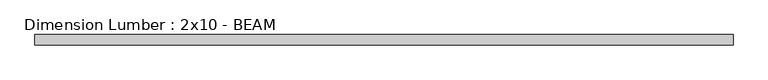
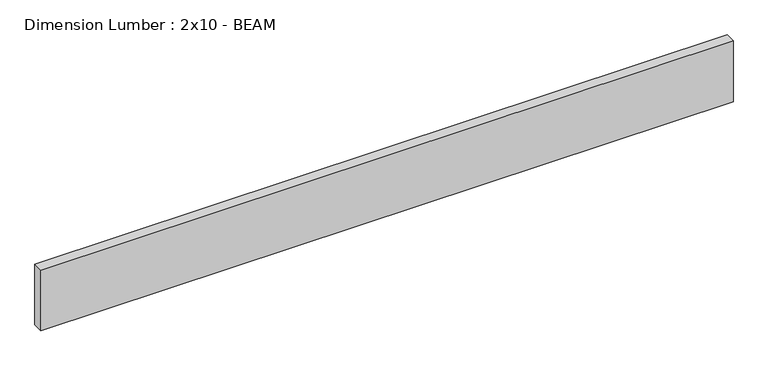
"""IFC4 building model written with IfcOpenShell, lengths in millimetres: beam geometry, Dimension Lumber : 2x10 - BEAM."""

from ifc_helpers import new_model, si_unit, frame, origin, place, context, project, spatial, polyline, outline, extrude, source, transform, mapped, element, save


def dimension_lumber_2x10_beam_c97c06ab(model_context):
    return source(origin(), model_context, "Body", "SweptSolid", [
        extrude(outline(polyline([(1213.64375, 19.05), (1213.64375, -19.05), (-1323.18125, -19.05), (-1323.18125, 19.05), (1213.64375, 19.05)])), frame((0.0, 0.0, -117.475), z_axis=(0.0, 0.0, 1.0), x_axis=(1.0, 0.0, 0.0)), (0.0, 0.0, 1.0), 234.95),
    ])


if __name__ == "__main__":
    model = new_model("IFC4")
    model_context = context("Model", 3, world=origin())
    ifc_project = project(units=[si_unit("LENGTHUNIT", "METRE", prefix="MILLI")], contexts=[model_context])
    site = spatial("IfcSite", under=ifc_project)
    building = spatial("IfcBuilding", under=site)
    placement = place(None, origin())
    dimension_lumber_2x10_beam_shape = dimension_lumber_2x10_beam_c97c06ab(model_context)
    element("IfcBeam", 1, ObjectType="Dimension Lumber : 2x10 - BEAM", at=placement, inside=building, context=model_context, shape_type="MappedRepresentation", body=[
        mapped(dimension_lumber_2x10_beam_shape, transform((0.0, 0.0, 0.0), x_axis=(1.0, 0.0, 0.0), y_axis=(0.0, 1.0, 0.0), z_axis=(0.0, 0.0, 1.0))),
    ])
    save(model, "model.ifc")

# Revit data of these elements
# Type "Dimension Lumber : 2x10 - BEAM"
#   Assembly Code = "B10"
#   A = 0.0755556 SF
#   Length [instance default] = 5' - 0"
#   b = 0' - 1 1/2"
#   d = 0' - 9 1/4"
#   Structural Material = (3) SISTERED 2X10s AT BEAM
# Element 1 (IfcBeam, "Dimension Lumber : 2x10 - BEAM")
#   Materials on its faces: "(3) SISTERED 2X10s AT BEAM"
# Materials
#   "(3) SISTERED 2X10s AT BEAM": class "Wood", colour RGB 234 198 147, transparency 0, Description = "Pinus Echinata", Cost = 0
